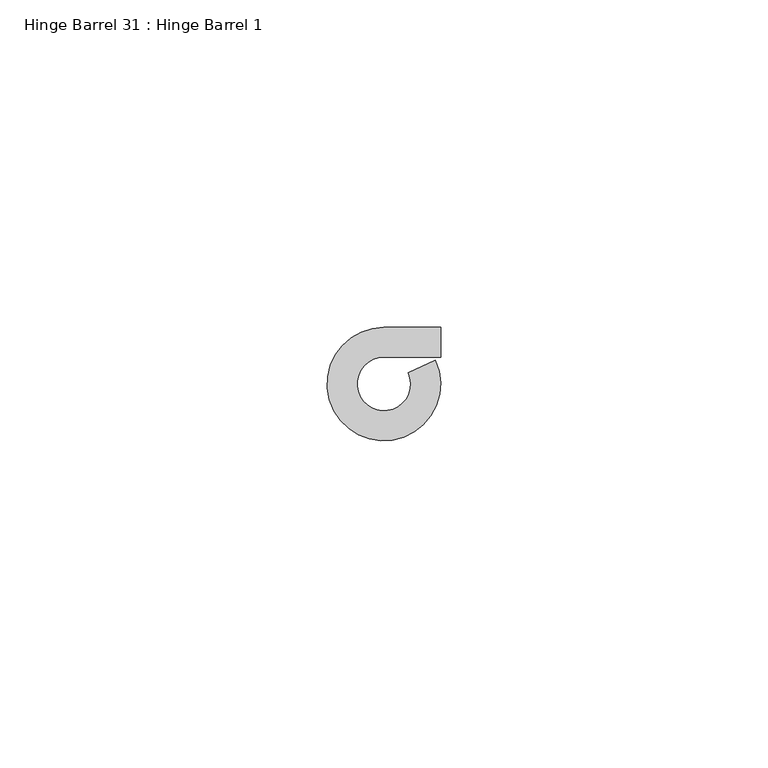
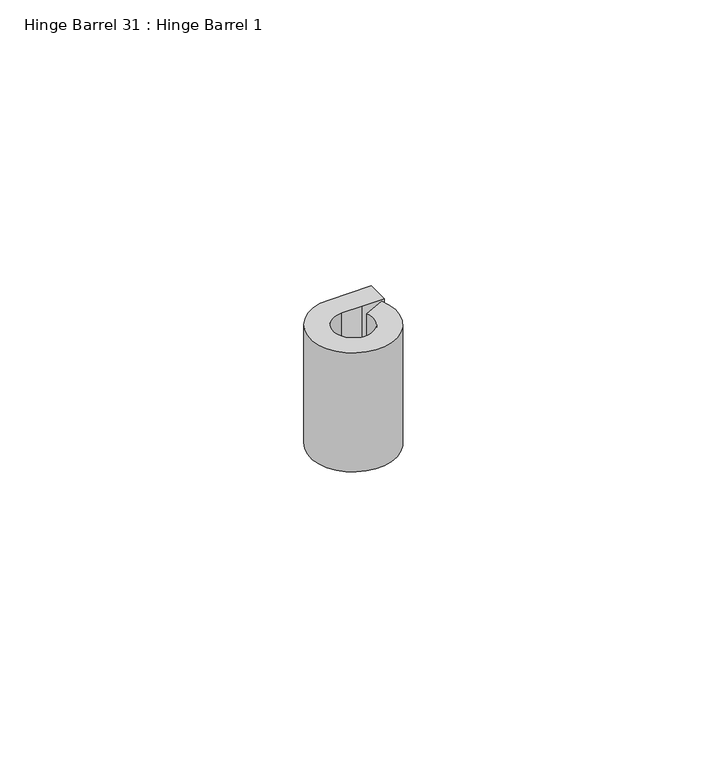
"""IFC4 building model written with IfcOpenShell, lengths in millimetres: proxy geometry, Hinge Barrel 31 : Hinge Barrel 1."""

from ifc_helpers import new_model, si_unit, point, frame, frame_2d, origin, place, context, project, spatial, polyline, circle_curve, trimmed, segment, composite_curve, outline, extrude, source, transform, mapped, element, save


def hinge_barrel_31_hinge_barrel_1_f2478639(model_context):
    return source(origin(), model_context, "Body", "SweptSolid", [
        extrude(outline(composite_curve([segment(polyline([(587323.2214739, -533980.5883841), (587319.1320739, -533980.5883841)]), True, "CONTINUOUS"), segment(trimmed(circle_curve(frame_2d((587319.1320739, -533984.6777841)), 4.0894), [point((587319.1320739, -533980.5883841))], [point((587322.8436736, -533982.9610371))], True, "CARTESIAN"), True, "CONTINUOUS"), segment(polyline([(587322.8436736, -533982.9610371), (587326.986084, -533981.0450249)]), True, "CONTINUOUS"), segment(trimmed(circle_curve(frame_2d((587319.1320739, -533984.6777841)), 8.6534625), [point((587326.986084, -533981.0450249))], [point((587319.1320739, -533976.0243216))], False, "CARTESIAN"), True, "CONTINUOUS"), segment(polyline([(587319.1320739, -533976.0243216), (587327.7934739, -533976.0243216), (587327.7934739, -533980.5883841), (587323.2214739, -533980.5883841)]), True, "CONTINUOUS")], self_intersect=False)), frame((0.0, 0.0, 1123.95), z_axis=(0.0, 0.0, 1.0), x_axis=(1.0, 0.0, 0.0)), (0.0, 0.0, 1.0), 25.4),
    ])


if __name__ == "__main__":
    model = new_model("IFC4")
    model_context = context("Model", 3, world=origin())
    ifc_project = project(units=[si_unit("LENGTHUNIT", "METRE", prefix="MILLI")], contexts=[model_context])
    site = spatial("IfcSite", under=ifc_project)
    building = spatial("IfcBuilding", under=site)
    placement = place(None, origin())
    hinge_barrel_31_hinge_barrel_1_shape = hinge_barrel_31_hinge_barrel_1_f2478639(model_context)
    element("IfcBuildingElementProxy", 1, Name="Hinge Barrel 31 : Hinge Barrel 1", ObjectType="Hinge Barrel 31 : Hinge Barrel 1", at=placement, inside=building, context=model_context, shape_type="MappedRepresentation", body=[
        mapped(hinge_barrel_31_hinge_barrel_1_shape, transform((0.0, 0.0, 0.0), x_axis=(1.0, 0.0, 0.0), y_axis=(0.0, 1.0, 0.0), z_axis=(0.0, 0.0, 1.0))),
    ])
    save(model, "model.ifc")

# Revit data of these elements
# Element 1 (IfcBuildingElementProxy, "Hinge Barrel 31 : Hinge Barrel 1")
#   Materials on its faces: "6\"X6\" WELD-ON STL BUTT HINGE"
# Materials
#   "6\"X6\" WELD-ON STL BUTT HINGE": class "Metal", colour RGB 189 187 185, transparency 0, Description = "Carbon steel", Cost = 0
